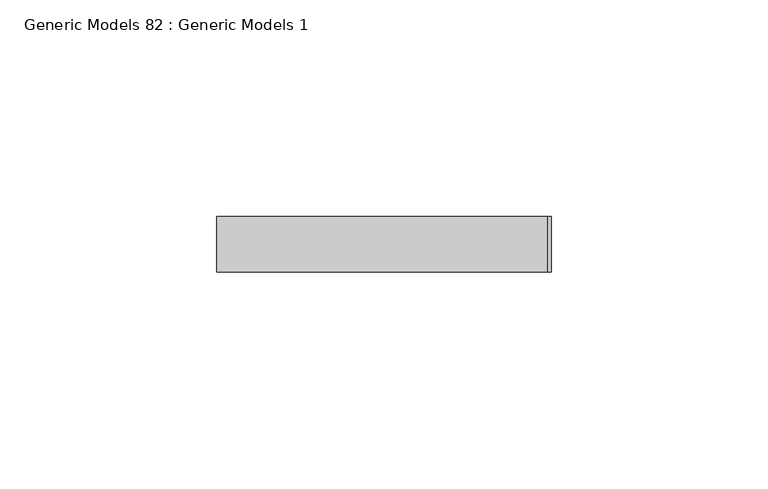
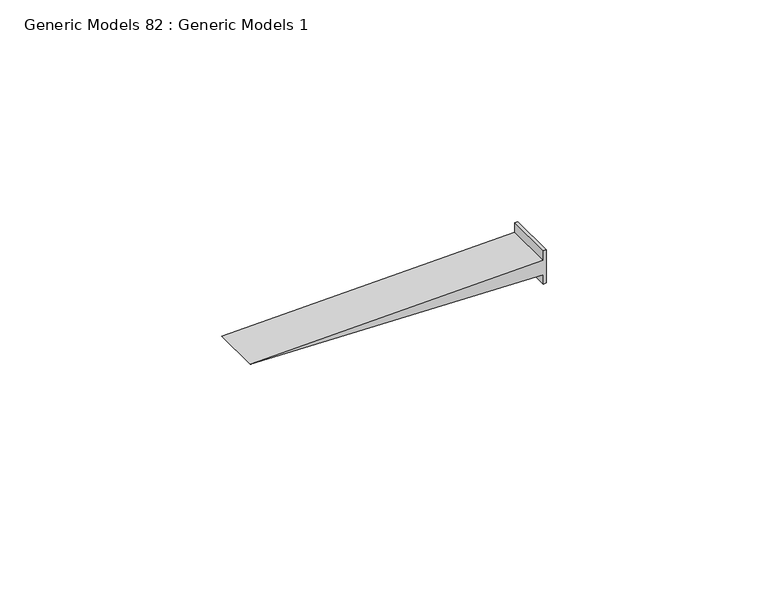
"""IFC4 building model written with IfcOpenShell, lengths in millimetres: proxy geometry, Generic Models 82 : Generic Models 1."""

from ifc_helpers import new_model, si_unit, frame, origin, place, context, project, spatial, polyline, outline, extrude, source, transform, mapped, element, save


def generic_models_82_generic_models_1_f14c7ad8(model_context):
    return source(origin(), model_context, "Body", "SweptSolid", [
        extrude(outline(polyline([(2442.2225782, 49800.66875), (2442.2225782, 49799.875), (2439.6727146, 49799.875), (2437.6759782, 49723.675), (2435.6792418, 49799.875), (2433.1293782, 49799.875), (2433.1293782, 49800.66875), (2442.2225782, 49800.66875)])), frame((0.0, 565.15, 0.0), z_axis=(0.0, 1.0, 0.0), x_axis=(0.0, 0.0, 1.0)), (0.0, 0.0, 1.0), 12.7),
    ])


if __name__ == "__main__":
    model = new_model("IFC4")
    model_context = context("Model", 3, world=origin())
    ifc_project = project(units=[si_unit("LENGTHUNIT", "METRE", prefix="MILLI")], contexts=[model_context])
    site = spatial("IfcSite", under=ifc_project)
    building = spatial("IfcBuilding", under=site)
    placement = place(None, origin())
    generic_models_82_generic_models_1_shape = generic_models_82_generic_models_1_f14c7ad8(model_context)
    element("IfcBuildingElementProxy", 1, Name="Generic Models 82 : Generic Models 1", ObjectType="Generic Models 82 : Generic Models 1", at=placement, inside=building, context=model_context, shape_type="MappedRepresentation", body=[
        mapped(generic_models_82_generic_models_1_shape, transform((0.0, 0.0, 0.0), x_axis=(1.0, 0.0, 0.0), y_axis=(0.0, 1.0, 0.0), z_axis=(0.0, 0.0, 1.0))),
    ])
    save(model, "model.ifc")

# Revit data of these elements
# Element 1 (IfcBuildingElementProxy, "Generic Models 82 : Generic Models 1")
#   Materials on its faces: "ATTACH GYPSUM BOARD TO STUDS AND NOT TO TOP TRACK"
# Materials
#   "ATTACH GYPSUM BOARD TO STUDS AND NOT TO TOP TRACK": class "Generic", colour RGB 48 48 48, transparency 0, Cost = 0
